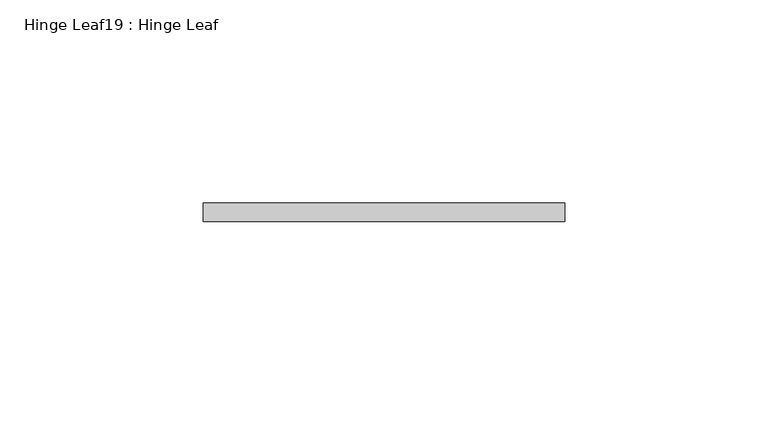
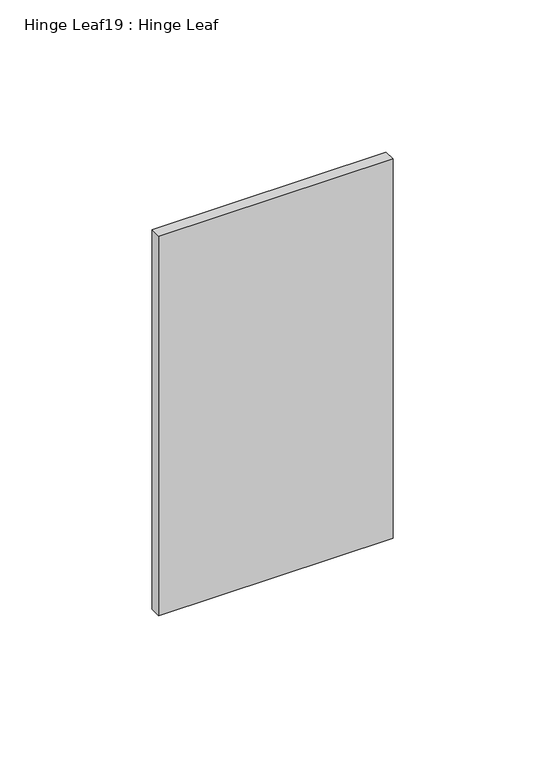
"""IFC4 building model written with IfcOpenShell, lengths in millimetres: proxy geometry, Hinge Leaf19 : Hinge Leaf."""

from ifc_helpers import new_model, si_unit, frame, origin, place, context, project, spatial, polyline, outline, extrude, source, transform, mapped, element, save


def hinge_leaf19_hinge_leaf_a46fc4d1(model_context):
    return source(origin(), model_context, "Body", "SweptSolid", [
        extrude(outline(polyline([(587327.7934739, -534096.6663841), (587416.6934739, -534096.6663841), (587416.6934739, -534101.2383841), (587327.7934739, -534101.2383841), (587327.7934739, -534096.6663841)])), frame((0.0, 0.0, 1123.95), z_axis=(0.0, 0.0, 1.0), x_axis=(1.0, 0.0, 0.0)), (0.0, 0.0, 1.0), 152.4),
    ])


if __name__ == "__main__":
    model = new_model("IFC4")
    model_context = context("Model", 3, world=origin())
    ifc_project = project(units=[si_unit("LENGTHUNIT", "METRE", prefix="MILLI")], contexts=[model_context])
    site = spatial("IfcSite", under=ifc_project)
    building = spatial("IfcBuilding", under=site)
    placement = place(None, origin())
    hinge_leaf19_hinge_leaf_shape = hinge_leaf19_hinge_leaf_a46fc4d1(model_context)
    element("IfcBuildingElementProxy", 1, Name="Hinge Leaf19 : Hinge Leaf", ObjectType="Hinge Leaf19 : Hinge Leaf", at=placement, inside=building, context=model_context, shape_type="MappedRepresentation", body=[
        mapped(hinge_leaf19_hinge_leaf_shape, transform((0.0, 0.0, 0.0), x_axis=(1.0, 0.0, 0.0), y_axis=(0.0, 1.0, 0.0), z_axis=(0.0, 0.0, 1.0))),
    ])
    save(model, "model.ifc")

# Revit data of these elements
# Element 1 (IfcBuildingElementProxy, "Hinge Leaf19 : Hinge Leaf")
#   Materials on its faces: "6\"X6\" WELD-ON STL BUTT HINGE"
# Materials
#   "6\"X6\" WELD-ON STL BUTT HINGE": class "Metal", colour RGB 189 187 185, transparency 0, Description = "Carbon steel", Cost = 0
